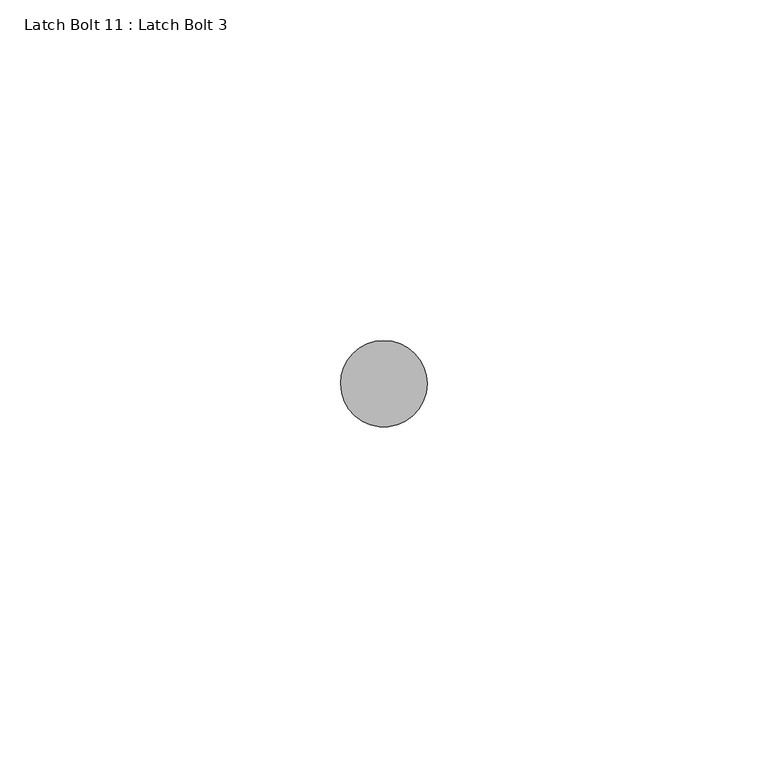
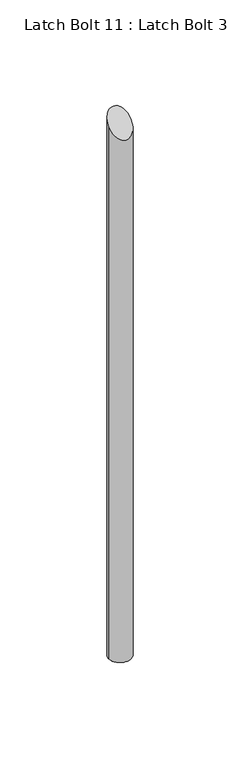
"""IFC4 building model written with IfcOpenShell, lengths in millimetres: proxy geometry, Latch Bolt 11 : Latch Bolt 3."""

from ifc_helpers import new_model, si_unit, frame, origin, place, context, project, spatial, circle_curve, ellipse_curve, source, transform, mapped, element, save
from ifc_brep_helpers import plane_surface, cylinder_surface, advanced_brep


def latch_bolt_11_latch_bolt_3_8ccbf98d(model_context):
    return source(origin(), model_context, "Body", "AdvancedBrep", [
        advanced_brep(
        [(587315.8935739, -532839.3663841, -25.4), (587303.1935739, -532839.3663841, -25.4), (587303.1935739, -532839.3663841, 292.0822144), (587309.5435739, -532833.0163841, 298.4322144), (587315.8935739, -532839.3663841, 292.0822144)],
        [
            (0, 1, circle_curve(frame((587309.5435739, -532839.3663841, -25.4), z_axis=(0.0, 0.0, -1.0), x_axis=(1.0, 0.0, 0.0)), 6.35)),
            (1, 0, circle_curve(frame((587309.5435739, -532839.3663841, -25.4), z_axis=(0.0, 0.0, -1.0), x_axis=(1.0, 0.0, 0.0)), 6.35)),
            (1, 2),
            (2, 3, ellipse_curve(frame((587309.5435739, -532839.3663841, 292.0822144), z_axis=(0.0, 0.7071067811865513, -0.7071067811865438), x_axis=(0.0, 0.7071067811865438, 0.7071067811865512)), 8.9802561, 6.35)),
            (3, 4, ellipse_curve(frame((587309.5435739, -532839.3663841, 292.0822144), z_axis=(0.0, 0.7071067811865513, -0.7071067811865438), x_axis=(0.0, 0.7071067811865438, 0.7071067811865512)), 8.9802561, 6.35)),
            (4, 0),
            (4, 2, ellipse_curve(frame((587309.5435739, -532839.3663841, 292.0822144), z_axis=(0.0, 0.7071067811865513, -0.7071067811865438), x_axis=(0.0, 0.7071067811865438, 0.7071067811865512)), 8.9802561, 6.35)),
        ],
        [
            plane_surface(frame((587315.8935739, -532839.3663841, -25.4), z_axis=(0.0, 0.0, -1.0), x_axis=(0.0, -1.0, 0.0))),
            cylinder_surface(frame((587309.5435739, -532839.3663841, -25.4), z_axis=(0.0, 0.0, 1.0), x_axis=(1.0, 0.0, 0.0)), 6.35),
            plane_surface(frame((587338.1185739, -532833.0163841, 298.4322144), z_axis=(0.0, -0.7071067811865513, 0.7071067811865438), x_axis=(-1.0, 0.0, 0.0))),
        ],
        [
            (0, [[1, 2]]),
            (1, [[-2, 3, 4, 5, 6]]),
            (1, [[-1, -6, 7, -3]]),
            (2, [[-5, -4, -7]]),
        ],
    ),
    ])


if __name__ == "__main__":
    model = new_model("IFC4")
    model_context = context("Model", 3, world=origin())
    ifc_project = project(units=[si_unit("LENGTHUNIT", "METRE", prefix="MILLI")], contexts=[model_context])
    site = spatial("IfcSite", under=ifc_project)
    building = spatial("IfcBuilding", under=site)
    placement = place(None, origin())
    latch_bolt_11_latch_bolt_3_shape = latch_bolt_11_latch_bolt_3_8ccbf98d(model_context)
    element("IfcBuildingElementProxy", 1, Name="Latch Bolt 11 : Latch Bolt 3", ObjectType="Latch Bolt 11 : Latch Bolt 3", at=placement, inside=building, context=model_context, shape_type="MappedRepresentation", body=[
        mapped(latch_bolt_11_latch_bolt_3_shape, transform((0.0, 0.0, 0.0), x_axis=(1.0, 0.0, 0.0), y_axis=(0.0, 1.0, 0.0), z_axis=(0.0, 0.0, 1.0))),
    ])
    save(model, "model.ifc")

# Revit data of these elements
# Element 1 (IfcBuildingElementProxy, "Latch Bolt 11 : Latch Bolt 3")
#   Materials on its faces: "GALV. SLIDE BOLT"
# Materials
#   "GALV. SLIDE BOLT": class "Metal", colour RGB 189 187 185, transparency 0, Description = "Carbon steel", Cost = 0
